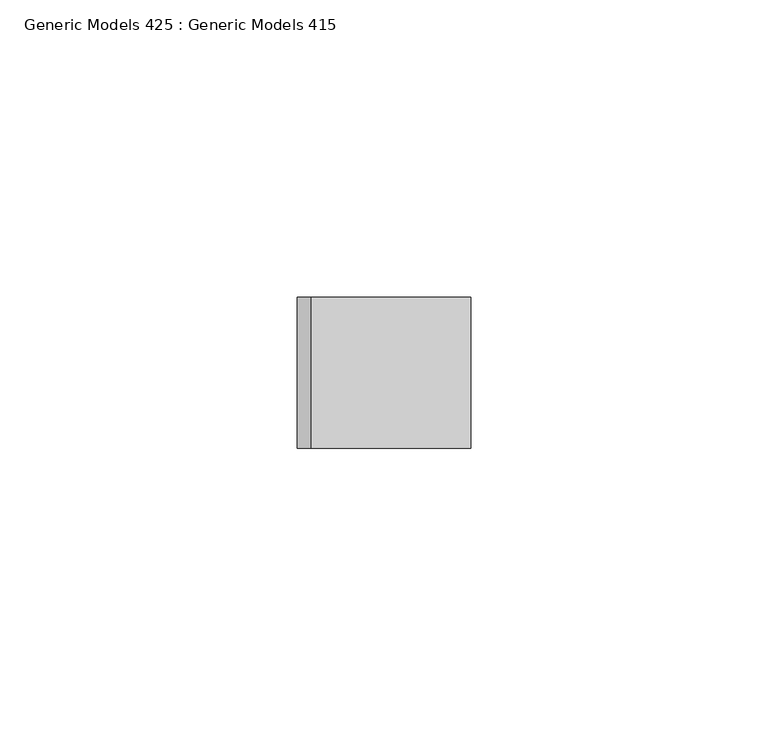
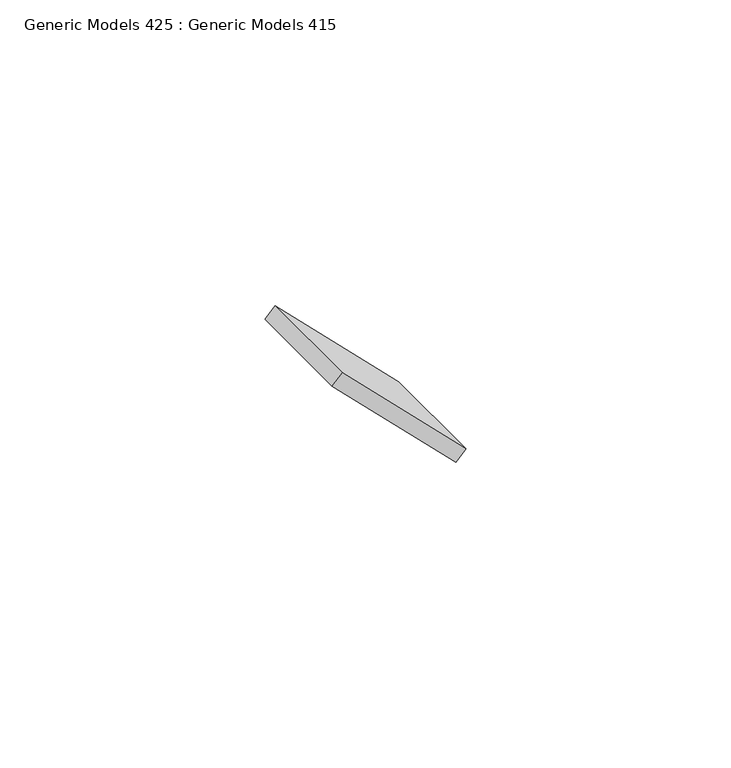
"""IFC4 building model written with IfcOpenShell, lengths in millimetres: proxy geometry, Generic Models 425 : Generic Models 415."""

from ifc_helpers import new_model, si_unit, frame, origin, place, context, project, spatial, polyline, outline, extrude, source, transform, mapped, element, save


def generic_models_425_generic_models_415_8684d8db(model_context):
    return source(origin(), model_context, "Body", "SweptSolid", [
        extrude(outline(polyline([(0.0, -38.1), (0.0, 0.0), (25.4, 0.0), (25.4, -38.1), (0.0, -38.1)])), frame((-6869.8996186, -4475.9863946, 128480.0002957), z_axis=(0.7071067811864907, 0.0, 0.7071067811866044), x_axis=(0.0, -1.0, 0.0)), (0.0, 0.0, 1.0), 3.175),
    ])


if __name__ == "__main__":
    model = new_model("IFC4")
    model_context = context("Model", 3, world=origin())
    ifc_project = project(units=[si_unit("LENGTHUNIT", "METRE", prefix="MILLI")], contexts=[model_context])
    site = spatial("IfcSite", under=ifc_project)
    building = spatial("IfcBuilding", under=site)
    placement = place(None, origin())
    generic_models_425_generic_models_415_shape = generic_models_425_generic_models_415_8684d8db(model_context)
    element("IfcBuildingElementProxy", 1, Name="Generic Models 425 : Generic Models 415", ObjectType="Generic Models 425 : Generic Models 415", at=placement, inside=building, context=model_context, shape_type="MappedRepresentation", body=[
        mapped(generic_models_425_generic_models_415_shape, transform((0.0, 0.0, 0.0), x_axis=(1.0, 0.0, 0.0), y_axis=(0.0, 1.0, 0.0), z_axis=(0.0, 0.0, 1.0))),
    ])
    save(model, "model.ifc")

# Revit data of these elements
# Element 1 (IfcBuildingElementProxy, "Generic Models 425 : Generic Models 415")
#   Materials on its faces: "_WELDED STEEL TABS FOR LOUVER ATTACHMENT"
# Materials
#   "_WELDED STEEL TABS FOR LOUVER ATTACHMENT": class "Metal", colour RGB 199 199 199, transparency 0, Description = "Structural steel 50ksi", Cost = 0
